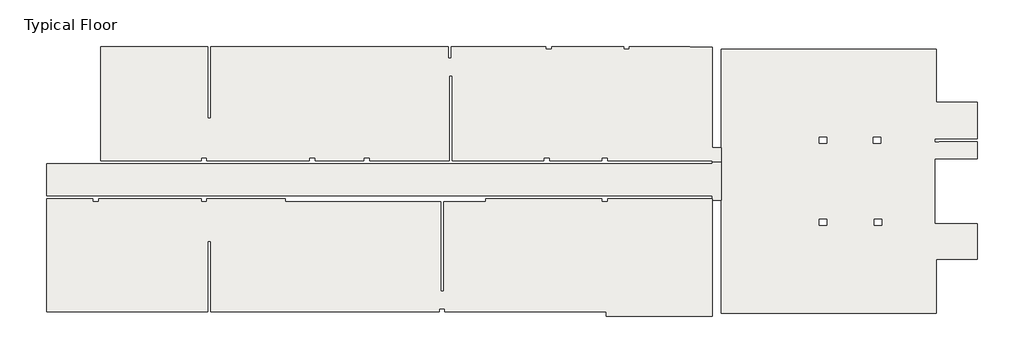
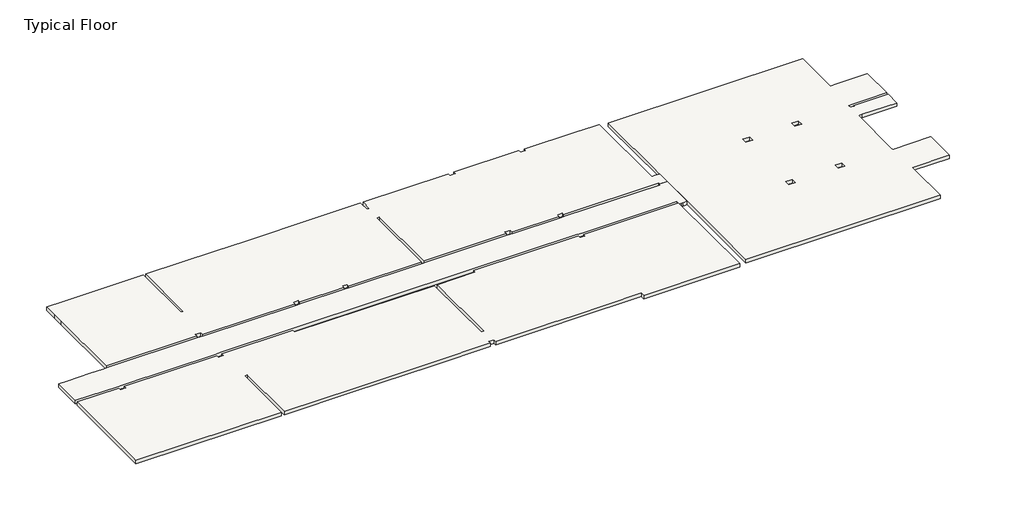
# One storey: 4 slabs.
"""IFC4 building model written with IfcOpenShell, lengths in millimetres."""

from ifc_helpers import new_model, si_unit, origin, place, context, project, spatial, faceted_brep, element, save

model = new_model("IFC4")

# Units and contexts
model_context = context("Model", 3, world=origin())
ifc_project = project(units=[si_unit("LENGTHUNIT", "METRE", prefix="MILLI")], contexts=[model_context])

# Site, building, storey
site = spatial("IfcSite", under=ifc_project)
building = spatial("IfcBuilding", under=site)
storey = spatial("IfcBuildingStorey", under=building, Name="Typical Floor", Elevation=4000.0)

# Slabs
placement = place(None, origin())
element("IfcSlab", 1, ObjectType="27", at=placement, inside=storey, context=model_context, shape_type="Brep", body=[
    faceted_brep([(37060.7744437, 13824.905611, 3730.0), (37060.7744437, 10224.905611, 3730.0), (37460.7744437, 10224.905611, 3730.0), (39861.089688, 10224.905611, 3730.0), (39861.089688, 7724.7029539, 3730.0), (37261.2473102, 7724.7029539, 3730.0), (36961.2473102, 7724.7029539, 3730.0), (36961.2473102, 7474.9393871, 3730.0), (37261.2473102, 7474.9393871, 3730.0), (37261.2473102, 7524.7029539, 3730.0), (39861.089688, 7524.7029539, 3730.0), (39861.089688, 6374.286381, 3730.0), (37261.2473102, 6374.286381, 3730.0), (36961.2473102, 6374.286381, 3730.0), (36961.2473102, 2122.9916276, 3730.0), (36961.2473102, 1922.9916276, 3730.0), (39861.089688, 1922.9916276, 3730.0), (39861.089688, -500.6066611, 3730.0), (37060.7294088, -500.6066611, 3730.0), (37060.7294088, -900.6066611, 3730.0), (37060.7294088, -4175.094389, 3730.0), (22360.0989202, -4175.094389, 3730.0), (22360.0989202, 3516.821846, 3730.0), (22360.0989202, 6129.9270025, 3730.0), (22360.0989202, 7129.9270025, 3730.0), (22360.0989202, 13824.905611, 3730.0), (33259.8287108, 7824.1850525, 3730.0), (32759.8287108, 7824.1850525, 3730.0), (32759.8287108, 7424.1850525, 3730.0), (33259.8287108, 7424.1850525, 3730.0), (29559.8287108, 7824.1850525, 3730.0), (29059.8287108, 7824.1850525, 3730.0), (29059.8287108, 7424.1850525, 3730.0), (29559.8287108, 7424.1850525, 3730.0), (29559.8287108, 2225.6261694, 3730.0), (29059.8287108, 2225.6261694, 3730.0), (29059.8287108, 1825.6261694, 3730.0), (29559.8287108, 1825.6261694, 3730.0), (33312.1592669, 2225.6261694, 3730.0), (32812.1592669, 2225.6261694, 3730.0), (32812.1592669, 1825.6261694, 3730.0), (33312.1592669, 1825.6261694, 3730.0), (37060.7744437, 10224.905611, 4000.0), (37060.7744437, 13824.905611, 4000.0), (22360.0989202, 13824.905611, 4000.0), (22360.0989202, 7129.9270025, 4000.0), (22360.0989202, 6129.9270025, 4000.0), (22360.0989202, 3516.821846, 4000.0), (22360.0989202, -4175.094389, 4000.0), (37060.7294088, -4175.094389, 4000.0), (37060.7294088, -900.6066611, 4000.0), (37060.7294088, -500.6066611, 4000.0), (39861.089688, -500.6066611, 4000.0), (39861.089688, 1922.9916276, 4000.0), (36961.2473102, 1922.9916276, 4000.0), (36961.2473102, 2122.9916276, 4000.0), (36961.2473102, 6374.286381, 4000.0), (37261.2473102, 6374.286381, 4000.0), (39861.089688, 6374.286381, 4000.0), (39861.089688, 7524.7029539, 4000.0), (37261.2473102, 7524.7029539, 4000.0), (37261.2473102, 7474.9393871, 4000.0), (36961.2473102, 7474.9393871, 4000.0), (36961.2473102, 7724.7029539, 4000.0), (37261.2473102, 7724.7029539, 4000.0), (39861.089688, 7724.7029539, 4000.0), (39861.089688, 10224.905611, 4000.0), (37460.7744437, 10224.905611, 4000.0), (29059.8287108, 7824.1850525, 4000.0), (29559.8287108, 7824.1850525, 4000.0), (29559.8287108, 7424.1850525, 4000.0), (29059.8287108, 7424.1850525, 4000.0), (32759.8287108, 7824.1850525, 4000.0), (33259.8287108, 7824.1850525, 4000.0), (33259.8287108, 7424.1850525, 4000.0), (32759.8287108, 7424.1850525, 4000.0), (32812.1592669, 2225.6261694, 4000.0), (33312.1592669, 2225.6261694, 4000.0), (33312.1592669, 1825.6261694, 4000.0), (32812.1592669, 1825.6261694, 4000.0), (29059.8287108, 2225.6261694, 4000.0), (29559.8287108, 2225.6261694, 4000.0), (29559.8287108, 1825.6261694, 4000.0), (29059.8287108, 1825.6261694, 4000.0)], [[[0, 1, 2, 3, 4, 5, 6, 7, 8, 9, 10, 11, 12, 13, 14, 15, 16, 17, 18, 19, 20, 21, 22, 23, 24, 25], [26, 27, 28, 29], [30, 31, 32, 33], [34, 35, 36, 37], [38, 39, 40, 41]], [[42, 43, 44, 45, 46, 47, 48, 49, 50, 51, 52, 53, 54, 55, 56, 57, 58, 59, 60, 61, 62, 63, 64, 65, 66, 67], [68, 69, 70, 71], [72, 73, 74, 75], [76, 77, 78, 79], [80, 81, 82, 83]], [[1, 0, 43, 42]], [[1, 42, 67, 66, 3, 2]], [[4, 3, 66, 65]], [[4, 65, 64, 63, 6, 5]], [[7, 6, 63, 62]], [[8, 7, 62, 61]], [[9, 8, 61, 60]], [[10, 9, 60, 59]], [[11, 10, 59, 58]], [[12, 11, 58, 57]], [[13, 12, 57, 56]], [[13, 56, 55, 54, 15, 14]], [[16, 15, 54, 53]], [[17, 16, 53, 52]], [[18, 17, 52, 51]], [[18, 51, 50, 49, 20, 19]], [[21, 20, 49, 48]], [[25, 24, 23, 22, 21, 48, 47, 46, 45, 44]], [[0, 25, 44, 43]], [[27, 26, 73, 72]], [[28, 27, 72, 75]], [[29, 28, 75, 74]], [[26, 29, 74, 73]], [[31, 30, 69, 68]], [[32, 31, 68, 71]], [[33, 32, 71, 70]], [[30, 33, 70, 69]], [[35, 34, 81, 80]], [[36, 35, 80, 83]], [[37, 36, 83, 82]], [[34, 37, 82, 81]], [[39, 38, 77, 76]], [[40, 39, 76, 79]], [[41, 40, 79, 78]], [[38, 41, 78, 77]]]),
])
element("IfcSlab", 2, ObjectType="27", at=placement, inside=storey, context=model_context, shape_type="Brep", body=[
    faceted_brep([(-19991.1958333, 12173.8810669, 3730.0), (-19991.1958333, 12973.9711367, 3730.0), (-19991.1958333, 14024.905611, 3730.0), (-18691.5786299, 14024.905611, 3730.0), (-12690.9031064, 14024.905611, 3730.0), (-12690.9031064, 9123.8022559, 3730.0), (-12490.9031064, 9123.8022559, 3730.0), (-12490.9031064, 14024.905611, 3730.0), (-7191.8713568, 14024.905611, 3730.0), (-4990.5653446, 14024.905611, 3730.0), (207.9034687, 14024.905611, 3730.0), (3733.1905662, 14024.905611, 3730.0), (3733.1905662, 13223.7347035, 3730.0), (3933.1905662, 13223.7347035, 3730.0), (3933.1905662, 14024.905611, 3730.0), (10383.8278101, 14024.905611, 3730.0), (10383.8278101, 13824.905611, 3730.0), (10783.8278101, 13824.905611, 3730.0), (10783.8278101, 14024.905611, 3730.0), (15703.8278101, 14024.905611, 3730.0), (15703.8278101, 13824.905611, 3730.0), (16103.8278101, 13824.905611, 3730.0), (16103.8278101, 14025.1420442, 3730.0), (20235.5548985, 14025.1420442, 3730.0), (20235.5548985, 13975.1420442, 3730.0), (21760.6168215, 13975.1420442, 3730.0), (21760.6168215, 7129.9270025, 3730.0), (21960.6168215, 7129.9270025, 3730.0), (22060.0989202, 7129.9270025, 3730.0), (22360.0989202, 7129.9270025, 3730.0), (22360.0989202, 6129.9270025, 3730.0), (21767.3630499, 6129.9270025, 3730.0), (21767.3630499, 6225.0407157, 3730.0), (14607.3630499, 6225.0407157, 3730.0), (14607.3630499, 6425.0407157, 3730.0), (14207.3630499, 6425.0407157, 3730.0), (14207.3630499, 6225.0407157, 3730.0), (10655.59543, 6225.0407157, 3730.0), (10655.59543, 6425.0407157, 3730.0), (10255.59543, 6425.0407157, 3730.0), (10255.59543, 6225.0407157, 3730.0), (4009.3896205, 6225.0407157, 3730.0), (4009.3896205, 12023.5995988, 3730.0), (3809.3896205, 12023.5995988, 3730.0), (3809.3896205, 6225.0407157, 3730.0), (-1642.0852726, 6225.0407157, 3730.0), (-1642.0852726, 6425.0407157, 3730.0), (-2042.0852726, 6425.0407157, 3730.0), (-2042.0852726, 6225.0407157, 3730.0), (-5341.9726853, 6225.0407157, 3730.0), (-5341.9726853, 6425.0407157, 3730.0), (-5741.9726853, 6425.0407157, 3730.0), (-5741.9726853, 6225.0407157, 3730.0), (-12741.7475108, 6225.0407157, 3730.0), (-12741.7475108, 6425.0407157, 3730.0), (-13141.7475108, 6425.0407157, 3730.0), (-13141.7475108, 6225.0407157, 3730.0), (-19991.1958333, 6225.0407157, 3730.0), (-19991.1958333, 12973.9711367, 4000.0), (-19991.1958333, 12173.8810669, 4000.0), (-19991.1958333, 6225.0407157, 4000.0), (-13141.7475108, 6225.0407157, 4000.0), (-13141.7475108, 6425.0407157, 4000.0), (-12741.7475108, 6425.0407157, 4000.0), (-12741.7475108, 6225.0407157, 4000.0), (-5741.9726853, 6225.0407157, 4000.0), (-5741.9726853, 6425.0407157, 4000.0), (-5341.9726853, 6425.0407157, 4000.0), (-5341.9726853, 6225.0407157, 4000.0), (-2042.0852726, 6225.0407157, 4000.0), (-2042.0852726, 6425.0407157, 4000.0), (-1642.0852726, 6425.0407157, 4000.0), (-1642.0852726, 6225.0407157, 4000.0), (3809.3896205, 6225.0407157, 4000.0), (3809.3896205, 12023.5995988, 4000.0), (4009.3896205, 12023.5995988, 4000.0), (4009.3896205, 6225.0407157, 4000.0), (10255.59543, 6225.0407157, 4000.0), (10255.59543, 6425.0407157, 4000.0), (10655.59543, 6425.0407157, 4000.0), (10655.59543, 6225.0407157, 4000.0), (14207.3630499, 6225.0407157, 4000.0), (14207.3630499, 6425.0407157, 4000.0), (14607.3630499, 6425.0407157, 4000.0), (14607.3630499, 6225.0407157, 4000.0), (21767.3630499, 6225.0407157, 4000.0), (21767.3630499, 6129.9270025, 4000.0), (22360.0989202, 6129.9270025, 4000.0), (22360.0989202, 7129.9270025, 4000.0), (22060.0989202, 7129.9270025, 4000.0), (21960.6168215, 7129.9270025, 4000.0), (21760.6168215, 7129.9270025, 4000.0), (21760.6168215, 13975.1420442, 4000.0), (20235.5548985, 13975.1420442, 4000.0), (20235.5548985, 14025.1420442, 4000.0), (16103.8278101, 14025.1420442, 4000.0), (16103.8278101, 13824.905611, 4000.0), (15703.8278101, 13824.905611, 4000.0), (15703.8278101, 14024.905611, 4000.0), (10783.8278101, 14024.905611, 4000.0), (10783.8278101, 13824.905611, 4000.0), (10383.8278101, 13824.905611, 4000.0), (10383.8278101, 14024.905611, 4000.0), (3933.1905662, 14024.905611, 4000.0), (3933.1905662, 13223.7347035, 4000.0), (3733.1905662, 13223.7347035, 4000.0), (3733.1905662, 14024.905611, 4000.0), (207.9034687, 14024.905611, 4000.0), (-4990.5653446, 14024.905611, 4000.0), (-7191.8713568, 14024.905611, 4000.0), (-12490.9031064, 14024.905611, 4000.0), (-12490.9031064, 9123.8022559, 4000.0), (-12690.9031064, 9123.8022559, 4000.0), (-12690.9031064, 14024.905611, 4000.0), (-18691.5786299, 14024.905611, 4000.0), (-19991.1958333, 14024.905611, 4000.0)], [[[0, 1, 2, 3, 4, 5, 6, 7, 8, 9, 10, 11, 12, 13, 14, 15, 16, 17, 18, 19, 20, 21, 22, 23, 24, 25, 26, 27, 28, 29, 30, 31, 32, 33, 34, 35, 36, 37, 38, 39, 40, 41, 42, 43, 44, 45, 46, 47, 48, 49, 50, 51, 52, 53, 54, 55, 56, 57]], [[58, 59, 60, 61, 62, 63, 64, 65, 66, 67, 68, 69, 70, 71, 72, 73, 74, 75, 76, 77, 78, 79, 80, 81, 82, 83, 84, 85, 86, 87, 88, 89, 90, 91, 92, 93, 94, 95, 96, 97, 98, 99, 100, 101, 102, 103, 104, 105, 106, 107, 108, 109, 110, 111, 112, 113, 114, 115]], [[1, 0, 59, 58]], [[2, 1, 58, 115]], [[2, 115, 114, 113, 4, 3]], [[5, 4, 113, 112]], [[6, 5, 112, 111]], [[7, 6, 111, 110]], [[7, 110, 109, 108, 107, 106, 11, 10, 9, 8]], [[12, 11, 106, 105]], [[13, 12, 105, 104]], [[14, 13, 104, 103]], [[15, 14, 103, 102]], [[16, 15, 102, 101]], [[17, 16, 101, 100]], [[18, 17, 100, 99]], [[19, 18, 99, 98]], [[20, 19, 98, 97]], [[21, 20, 97, 96]], [[22, 21, 96, 95]], [[23, 22, 95, 94]], [[24, 23, 94, 93]], [[25, 24, 93, 92]], [[26, 25, 92, 91]], [[26, 91, 90, 89, 88, 29, 28, 27]], [[30, 29, 88, 87]], [[31, 30, 87, 86]], [[32, 31, 86, 85]], [[33, 32, 85, 84]], [[34, 33, 84, 83]], [[35, 34, 83, 82]], [[36, 35, 82, 81]], [[37, 36, 81, 80]], [[38, 37, 80, 79]], [[39, 38, 79, 78]], [[40, 39, 78, 77]], [[41, 40, 77, 76]], [[42, 41, 76, 75]], [[43, 42, 75, 74]], [[44, 43, 74, 73]], [[45, 44, 73, 72]], [[46, 45, 72, 71]], [[47, 46, 71, 70]], [[48, 47, 70, 69]], [[49, 48, 69, 68]], [[50, 49, 68, 67]], [[51, 50, 67, 66]], [[52, 51, 66, 65]], [[53, 52, 65, 64]], [[54, 53, 64, 63]], [[55, 54, 63, 62]], [[56, 55, 62, 61]], [[57, 56, 61, 60]], [[0, 57, 60, 59]]]),
])
element("IfcSlab", 3, ObjectType="27", at=placement, inside=storey, context=model_context, shape_type="Brep", body=[
    faceted_brep([(21767.3630499, 6025.0407157, 3730.0), (21767.3630499, 6129.9270025, 3730.0), (22360.0989202, 6129.9270025, 3730.0), (22360.0989202, 3516.821846, 3730.0), (22060.0989202, 3516.821846, 3730.0), (21960.6168215, 3516.821846, 3730.0), (21960.6168215, 3525.2884076, 3730.0), (21760.6168215, 3525.2884076, 3730.0), (21760.6168215, 3625.8513439, 3730.0), (21767.3630499, 3625.8513439, 3730.0), (21767.3630499, 3825.8513439, 3730.0), (14607.3630499, 3825.8513439, 3730.0), (14207.3630499, 3825.8513439, 3730.0), (6309.1644459, 3825.8513439, 3730.0), (-7390.8355541, 3825.8513439, 3730.0), (-12741.7475108, 3825.8513439, 3730.0), (-13141.7475108, 3825.8513439, 3730.0), (-20137.3553255, 3825.8513439, 3730.0), (-20537.3553255, 3825.8513439, 3730.0), (-23692.1640837, 3825.8513439, 3730.0), (-23692.1640837, 6025.0407157, 3730.0), (-23092.0740139, 6025.0407157, 3730.0), (-21341.6124061, 6025.0407157, 3730.0), (-20240.9594, 6025.0407157, 3730.0), (-19991.1958333, 6025.0407157, 3730.0), (-13141.7475108, 6025.0407157, 3730.0), (-12741.7475108, 6025.0407157, 3730.0), (-5741.9726853, 6025.0407157, 3730.0), (-5341.9726853, 6025.0407157, 3730.0), (-2042.0852726, 6025.0407157, 3730.0), (-1642.0852726, 6025.0407157, 3730.0), (3809.3896205, 6025.0407157, 3730.0), (4009.3896205, 6025.0407157, 3730.0), (10255.59543, 6025.0407157, 3730.0), (10655.59543, 6025.0407157, 3730.0), (14207.3630499, 6025.0407157, 3730.0), (14607.3630499, 6025.0407157, 3730.0), (21767.3630499, 6129.9270025, 4000.0), (21767.3630499, 6025.0407157, 4000.0), (14607.3630499, 6025.0407157, 4000.0), (14207.3630499, 6025.0407157, 4000.0), (10655.59543, 6025.0407157, 4000.0), (10255.59543, 6025.0407157, 4000.0), (4009.3896205, 6025.0407157, 4000.0), (3809.3896205, 6025.0407157, 4000.0), (-1642.0852726, 6025.0407157, 4000.0), (-2042.0852726, 6025.0407157, 4000.0), (-5341.9726853, 6025.0407157, 4000.0), (-5741.9726853, 6025.0407157, 4000.0), (-12741.7475108, 6025.0407157, 4000.0), (-13141.7475108, 6025.0407157, 4000.0), (-19991.1958333, 6025.0407157, 4000.0), (-20240.9594, 6025.0407157, 4000.0), (-21341.6124061, 6025.0407157, 4000.0), (-23092.0740139, 6025.0407157, 4000.0), (-23692.1640837, 6025.0407157, 4000.0), (-23692.1640837, 3825.8513439, 4000.0), (-20537.3553255, 3825.8513439, 4000.0), (-20137.3553255, 3825.8513439, 4000.0), (-13141.7475108, 3825.8513439, 4000.0), (-12741.7475108, 3825.8513439, 4000.0), (-7390.8355541, 3825.8513439, 4000.0), (6309.1644459, 3825.8513439, 4000.0), (14207.3630499, 3825.8513439, 4000.0), (14607.3630499, 3825.8513439, 4000.0), (21767.3630499, 3825.8513439, 4000.0), (21767.3630499, 3625.8513439, 4000.0), (21760.6168215, 3625.8513439, 4000.0), (21760.6168215, 3525.2884076, 4000.0), (21960.6168215, 3525.2884076, 4000.0), (21960.6168215, 3516.821846, 4000.0), (22060.0989202, 3516.821846, 4000.0), (22360.0989202, 3516.821846, 4000.0), (22360.0989202, 6129.9270025, 4000.0)], [[[0, 1, 2, 3, 4, 5, 6, 7, 8, 9, 10, 11, 12, 13, 14, 15, 16, 17, 18, 19, 20, 21, 22, 23, 24, 25, 26, 27, 28, 29, 30, 31, 32, 33, 34, 35, 36]], [[37, 38, 39, 40, 41, 42, 43, 44, 45, 46, 47, 48, 49, 50, 51, 52, 53, 54, 55, 56, 57, 58, 59, 60, 61, 62, 63, 64, 65, 66, 67, 68, 69, 70, 71, 72, 73]], [[1, 0, 38, 37]], [[2, 1, 37, 73]], [[3, 2, 73, 72]], [[4, 3, 72, 71]], [[5, 4, 71, 70]], [[6, 5, 70, 69]], [[7, 6, 69, 68]], [[8, 7, 68, 67]], [[9, 8, 67, 66]], [[10, 9, 66, 65]], [[10, 65, 64, 63, 62, 61, 60, 59, 58, 57, 56, 19, 18, 17, 16, 15, 14, 13, 12, 11]], [[20, 19, 56, 55]], [[20, 55, 54, 53, 52, 51, 50, 49, 48, 47, 46, 45, 44, 43, 42, 41, 40, 39, 38, 0, 36, 35, 34, 33, 32, 31, 30, 29, 28, 27, 26, 25, 24, 23, 22, 21]]]),
])
element("IfcSlab", 4, ObjectType="27", at=placement, inside=storey, context=model_context, shape_type="Brep", body=[
    faceted_brep([(-23692.1640837, -4074.5314528, 3730.0), (-23692.1640837, 3625.8513439, 3730.0), (-20537.3553255, 3625.8513439, 3730.0), (-20537.3553255, 3425.8513439, 3730.0), (-20137.3553255, 3425.8513439, 3730.0), (-20137.3553255, 3625.8513439, 3730.0), (-13141.7475108, 3625.8513439, 3730.0), (-13141.7475108, 3425.806309, 3730.0), (-12741.7475108, 3425.806309, 3730.0), (-12741.7475108, 3625.806309, 3730.0), (-7390.8355541, 3625.806309, 3730.0), (-7390.8355541, 3425.806309, 3730.0), (3209.2995507, 3425.806309, 3730.0), (3209.2995507, -2674.3513132, 3730.0), (3409.2995507, -2674.3513132, 3730.0), (3409.2995507, 3425.806309, 3730.0), (6309.1644459, 3425.806309, 3730.0), (6309.1644459, 3625.806309, 3730.0), (14207.3630499, 3625.806309, 3730.0), (14207.3630499, 3425.806309, 3730.0), (14607.3630499, 3425.806309, 3730.0), (14607.3630499, 3625.8513439, 3730.0), (21760.6168215, 3625.8513439, 3730.0), (21760.6168215, 3525.2884076, 3730.0), (21760.6168215, -4375.094389, 3730.0), (14509.4796903, -4375.094389, 3730.0), (14509.4796903, -4075.5672555, 3730.0), (14509.4796903, -4074.5314528, 3730.0), (9358.1399019, -4074.5314528, 3730.0), (7709.2770332, -4074.5314528, 3730.0), (3509.817452, -4074.5314528, 3730.0), (3509.817452, -3874.5314528, 3730.0), (3109.817452, -3874.5314528, 3730.0), (3109.817452, -4074.5314528, 3730.0), (-1290.6779319, -4074.5314528, 3730.0), (-7191.8713568, -4074.5314528, 3730.0), (-12491.9389092, -4074.5314528, 3730.0), (-12491.9389092, 724.9731633, 3730.0), (-12691.9389092, 724.9731633, 3730.0), (-12691.9389092, -4074.5314528, 3730.0), (-19792.231636, -4074.5314528, 3730.0), (-23692.1640837, 3625.8513439, 4000.0), (-23692.1640837, -4074.5314528, 4000.0), (-19792.231636, -4074.5314528, 4000.0), (-12691.9389092, -4074.5314528, 4000.0), (-12691.9389092, 724.9731633, 4000.0), (-12491.9389092, 724.9731633, 4000.0), (-12491.9389092, -4074.5314528, 4000.0), (-7191.8713568, -4074.5314528, 4000.0), (-1290.6779319, -4074.5314528, 4000.0), (3109.817452, -4074.5314528, 4000.0), (3109.817452, -3874.5314528, 4000.0), (3509.817452, -3874.5314528, 4000.0), (3509.817452, -4074.5314528, 4000.0), (7709.2770332, -4074.5314528, 4000.0), (9358.1399019, -4074.5314528, 4000.0), (14509.4796903, -4074.5314528, 4000.0), (14509.4796903, -4075.5672555, 4000.0), (14509.4796903, -4375.094389, 4000.0), (21760.6168215, -4375.094389, 4000.0), (21760.6168215, 3525.2884076, 4000.0), (21760.6168215, 3625.8513439, 4000.0), (14607.3630499, 3625.8513439, 4000.0), (14607.3630499, 3425.806309, 4000.0), (14207.3630499, 3425.806309, 4000.0), (14207.3630499, 3625.806309, 4000.0), (6309.1644459, 3625.806309, 4000.0), (6309.1644459, 3425.806309, 4000.0), (3409.2995507, 3425.806309, 4000.0), (3409.2995507, -2674.3513132, 4000.0), (3209.2995507, -2674.3513132, 4000.0), (3209.2995507, 3425.806309, 4000.0), (-7390.8355541, 3425.806309, 4000.0), (-7390.8355541, 3625.806309, 4000.0), (-12741.7475108, 3625.806309, 4000.0), (-12741.7475108, 3425.806309, 4000.0), (-13141.7475108, 3425.806309, 4000.0), (-13141.7475108, 3625.8513439, 4000.0), (-20137.3553255, 3625.8513439, 4000.0), (-20137.3553255, 3425.8513439, 4000.0), (-20537.3553255, 3425.8513439, 4000.0), (-20537.3553255, 3625.8513439, 4000.0)], [[[0, 1, 2, 3, 4, 5, 6, 7, 8, 9, 10, 11, 12, 13, 14, 15, 16, 17, 18, 19, 20, 21, 22, 23, 24, 25, 26, 27, 28, 29, 30, 31, 32, 33, 34, 35, 36, 37, 38, 39, 40]], [[41, 42, 43, 44, 45, 46, 47, 48, 49, 50, 51, 52, 53, 54, 55, 56, 57, 58, 59, 60, 61, 62, 63, 64, 65, 66, 67, 68, 69, 70, 71, 72, 73, 74, 75, 76, 77, 78, 79, 80, 81]], [[1, 0, 42, 41]], [[2, 1, 41, 81]], [[3, 2, 81, 80]], [[4, 3, 80, 79]], [[5, 4, 79, 78]], [[6, 5, 78, 77]], [[7, 6, 77, 76]], [[8, 7, 76, 75]], [[9, 8, 75, 74]], [[10, 9, 74, 73]], [[11, 10, 73, 72]], [[12, 11, 72, 71]], [[13, 12, 71, 70]], [[14, 13, 70, 69]], [[15, 14, 69, 68]], [[16, 15, 68, 67]], [[17, 16, 67, 66]], [[18, 17, 66, 65]], [[19, 18, 65, 64]], [[20, 19, 64, 63]], [[21, 20, 63, 62]], [[22, 21, 62, 61]], [[22, 61, 60, 59, 24, 23]], [[25, 24, 59, 58]], [[25, 58, 57, 56, 27, 26]], [[27, 56, 55, 54, 53, 30, 29, 28]], [[31, 30, 53, 52]], [[32, 31, 52, 51]], [[33, 32, 51, 50]], [[33, 50, 49, 48, 47, 36, 35, 34]], [[37, 36, 47, 46]], [[38, 37, 46, 45]], [[39, 38, 45, 44]], [[39, 44, 43, 42, 0, 40]]]),
])

save(model, "model.ifc")

# Revit data of these elements
# Type "27"
#   Function = 0
#   Layers, outside or top first: 27 cm "Concrete" (function 1)
# Element 1 (IfcSlab, "27")
#   Mark = "S1"
#   SOFiSTiK_AMG_Comments = ""
#   Height Offset From Level = 0 cm
#   built-in parameter 1001954 = 1
#   SOFiSTiK_AMG_Scheduled = yes
#   SOFiSTiK_AMG_Adjusted = yes
#   Phase Created = New Construction
#   Materials on its faces: "Concrete"
# Element 2 (IfcSlab, "27")
#   Mark = "S2"
#   SOFiSTiK_AMG_Comments = ""
#   built-in parameter 1001955 = 1.5708 (stored number, unit not read)
#   Height Offset From Level = 0 cm
#   built-in parameter 1001954 = 1
#   SOFiSTiK_AMG_Scheduled = yes
#   SOFiSTiK_AMG_Adjusted = no
#   Phase Created = New Construction
#   Materials on its faces: "Concrete"
# Element 3 (IfcSlab, "27")
#   Mark = "S3"
#   SOFiSTiK_AMG_Comments = ""
#   Height Offset From Level = 0 cm
#   built-in parameter 1001954 = 1
#   SOFiSTiK_AMG_Scheduled = yes
#   SOFiSTiK_AMG_Adjusted = no
#   Phase Created = New Construction
#   Materials on its faces: "Concrete"
# Element 4 (IfcSlab, "27")
#   Mark = "S4"
#   SOFiSTiK_AMG_Comments = ""
#   built-in parameter 1001955 = -1.5708 (stored number, unit not read)
#   Height Offset From Level = 0 cm
#   built-in parameter 1001954 = 1
#   SOFiSTiK_AMG_Scheduled = yes
#   SOFiSTiK_AMG_Adjusted = no
#   Phase Created = New Construction
#   Materials on its faces: "Concrete"
# Materials
#   "Concrete": class "Concrete", colour RGB 192 192 192, transparency 0, Keynote = "01000", Description = "Cast-in-place concrete", Cost = 0
